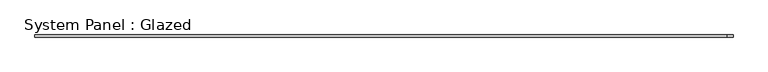
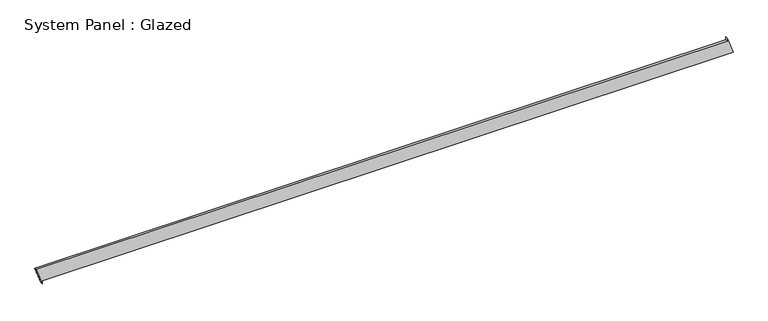
"""IFC4 building model written with IfcOpenShell, lengths in millimetres: plate geometry, System Panel : Glazed."""

from ifc_helpers import new_model, si_unit, frame, origin, place, context, project, spatial, polyline, outline, extrude, source, transform, mapped, element, save


def system_panel_glazed_1e3ff095(model_context):
    return source(origin(), model_context, "Body", "SweptSolid", [
        extrude(outline(polyline([(0.0, -3957.6016429), (35.3553391, -3957.6016429), (35.3553391, 4027.0288897), (234.5792262, 3957.9376669), (199.2238871, 3957.9382884), (199.0835123, -4027.0288897), (0.0, -3957.6016429)])), frame((0.0, -49.5, 0.0), z_axis=(0.0, 1.0, 0.0), x_axis=(0.0, 0.0, 1.0)), (0.0, 0.0, 1.0), 25.0),
    ])


if __name__ == "__main__":
    model = new_model("IFC4")
    model_context = context("Model", 3, world=origin())
    ifc_project = project(units=[si_unit("LENGTHUNIT", "METRE", prefix="MILLI")], contexts=[model_context])
    site = spatial("IfcSite", under=ifc_project)
    building = spatial("IfcBuilding", under=site)
    placement = place(None, origin())
    system_panel_glazed_shape = system_panel_glazed_1e3ff095(model_context)
    element("IfcPlate", 1, ObjectType="System Panel : Glazed", at=placement, inside=building, context=model_context, shape_type="MappedRepresentation", body=[
        mapped(system_panel_glazed_shape, transform((0.0, 0.0, 0.0), x_axis=(1.0, 0.0, 0.0), y_axis=(0.0, 1.0, 0.0), z_axis=(0.0, 0.0, 1.0))),
    ])
    save(model, "model.ifc")

# Revit data of these elements
# Element 1 (IfcPlate, "System Panel : Glazed")
#   Materials on its faces: "Glass"
# Materials
#   "Glass": class "Glass", colour RGB 218 227 224, transparency 0.85, Description = "Soda Lime Glass", Cost = 0
